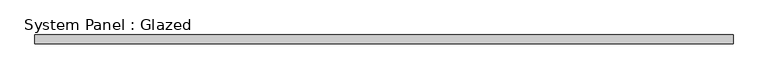
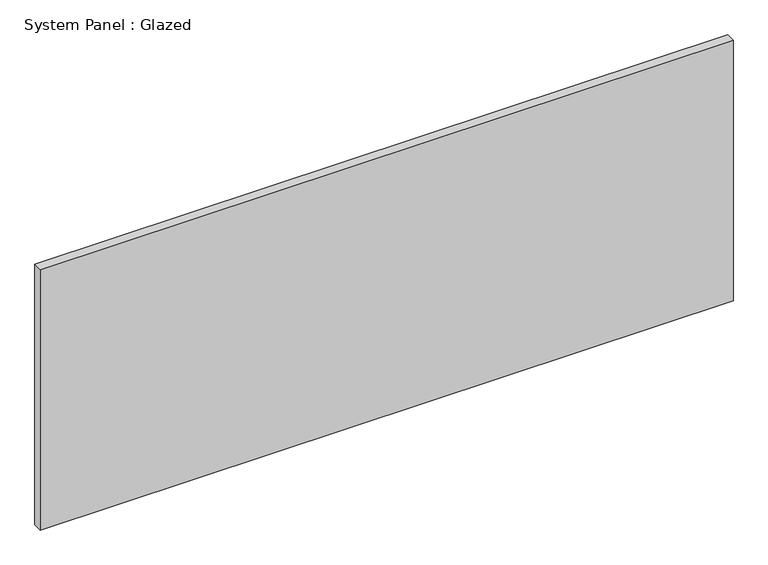
"""IFC4 building model written with IfcOpenShell, lengths in millimetres: plate geometry, System Panel : Glazed."""

import ifcopenshell
import ifcopenshell.guid

model = None  # the IFC model being written
_history = None  # IfcOwnerHistory: only IFC2X3 demands one
_inside = {}  # id of a spatial element -> (the spatial element, [elements in it])
_under = {}  # id of a project, library or spatial element -> (it, [spatial elements below it])
_declared = {}  # id of a project -> (the project, [libraries it declares])
_typed = {}  # id of a type object -> (the type object, [elements of that type])
_made_of = {}  # id of a material, layer set ... -> (it, [elements and type objects made of it])


def new_model(schema):
    """Start an empty IFC model of exactly this schema.

    Asked for "IFC4X3", IfcOpenShell would pick the latest addendum, in which some entities
    have other attributes; the version numbers below select the first issue.
    IFC2X3 requires an IfcOwnerHistory on every rooted entity: one is made here for all.
    """
    global model, _history
    if schema == "IFC4X3":
        model = ifcopenshell.file(schema_version=(4, 3, 0, 0))
    else:
        model = ifcopenshell.file(schema=schema)
    _inside.clear()
    _under.clear()
    _declared.clear()
    _typed.clear()
    _made_of.clear()
    _history = None
    if model.schema == "IFC2X3":
        org = make("IfcOrganization", Name="unknown")
        user = make(
            "IfcPersonAndOrganization",
            ThePerson=make("IfcPerson", FamilyName="unknown"),
            TheOrganization=org,
        )
        app = make(
            "IfcApplication",
            ApplicationDeveloper=org,
            Version="unknown",
            ApplicationFullName="unknown",
            ApplicationIdentifier="unknown",
        )
        _history = make(
            "IfcOwnerHistory",
            OwningUser=user,
            OwningApplication=app,
            ChangeAction="ADDED",
            CreationDate=0,
        )
    return model


def make(cls, **values):
    """One entity of the class cls with the attributes given. An attribute that is None is left unset."""
    return model.create_entity(
        cls, **{name: value for name, value in values.items() if value is not None}
    )


def rooted(cls, **values):
    """An entity with a GlobalId (a new one), such as an element, a storey or a relation."""
    return make(cls, GlobalId=ifcopenshell.guid.new(), OwnerHistory=_history, **values)


def si_unit(unit_type, name, prefix=None):
    """IfcSIUnit, for example si_unit("LENGTHUNIT", "METRE", prefix="MILLI")."""
    return make("IfcSIUnit", UnitType=unit_type, Prefix=prefix, Name=name)


def assignment(units):
    """IfcUnitAssignment: the units of a project."""
    return None if units is None else make("IfcUnitAssignment", Units=units)


def point(xyz):
    """IfcCartesianPoint."""
    return None if xyz is None else make("IfcCartesianPoint", Coordinates=xyz)


def direction(xyz):
    """IfcDirection."""
    return None if xyz is None else make("IfcDirection", DirectionRatios=xyz)


def frame(location, z_axis=None, x_axis=None):
    """IfcAxis2Placement3D, a coordinate frame: its origin and axes. An axis left out is left unset."""
    return make(
        "IfcAxis2Placement3D",
        Location=point(location),
        Axis=direction(z_axis),
        RefDirection=direction(x_axis),
    )


def origin():
    """The frame at (0, 0, 0) with its axes left unset."""
    return frame((0.0, 0.0, 0.0))


def origin_with_axes():
    """The frame at (0, 0, 0) with the z axis (0, 0, 1) and the x axis (1, 0, 0) written out."""
    return frame((0.0, 0.0, 0.0), z_axis=(0.0, 0.0, 1.0), x_axis=(1.0, 0.0, 0.0))


def place(relative_to, where):
    """IfcLocalPlacement: puts the frame where relative to a parent placement (None: the world)."""
    return make(
        "IfcLocalPlacement", PlacementRelTo=relative_to, RelativePlacement=where
    )


def context(
    kind, dimensions, precision=None, world=None, true_north=None, identifier=None
):
    """IfcGeometricRepresentationContext, for example the 3D "Model" context."""
    return make(
        "IfcGeometricRepresentationContext",
        ContextIdentifier=identifier,
        ContextType=kind,
        CoordinateSpaceDimension=dimensions,
        Precision=precision,
        WorldCoordinateSystem=world,
        TrueNorth=true_north,
    )


def project(units=None, contexts=None):
    """IfcProject with its units and contexts."""
    return rooted(
        "IfcProject",
        Name="project",
        RepresentationContexts=contexts,
        UnitsInContext=assignment(units),
    )


def spatial(cls, under=None, at=None, **own):
    """A site, building, storey or space (cls), placed at a placement, below another one or the project."""
    s = rooted(cls, ObjectPlacement=at, **own)
    if under is not None:
        _under.setdefault(under.id(), (under, []))[1].append(s)
    return s


def polyline(points):
    """IfcPolyline through the points."""
    return make("IfcPolyline", Points=[point(p) for p in points])


def outline(outer, holes=None, kind="AREA"):
    """IfcArbitraryClosedProfileDef: a profile drawn as a closed curve; with holes, ...WithVoids."""
    if holes is None:
        return make("IfcArbitraryClosedProfileDef", ProfileType=kind, OuterCurve=outer)
    return make(
        "IfcArbitraryProfileDefWithVoids",
        ProfileType=kind,
        OuterCurve=outer,
        InnerCurves=holes,
    )


def extrude(swept, where, along, depth):
    """IfcExtrudedAreaSolid: the profile swept, set in the frame where, extruded along a direction by depth."""
    return make(
        "IfcExtrudedAreaSolid",
        SweptArea=swept,
        Position=where,
        ExtrudedDirection=direction(along),
        Depth=depth,
    )


def shape(context_of_items, identifier, shape_type, items):
    """IfcShapeRepresentation: the items that make up one representation, for example the "Body"."""
    return make(
        "IfcShapeRepresentation",
        ContextOfItems=context_of_items,
        RepresentationIdentifier=identifier,
        RepresentationType=shape_type,
        Items=items,
    )


def source(mapping_origin, context_of_items, identifier, shape_type, items):
    """IfcRepresentationMap: a shape defined once, which mapped items show again and again."""
    return make(
        "IfcRepresentationMap",
        MappingOrigin=mapping_origin,
        MappedRepresentation=shape(context_of_items, identifier, shape_type, items),
    )


def transform(
    local_origin,
    x_axis=None,
    y_axis=None,
    z_axis=None,
    scale=None,
    scale2=None,
    scale3=None,
    uniform=True,
):
    """IfcCartesianTransformationOperator3D, or its non-uniform kind. x_axis, y_axis, z_axis: its Axis1, 2, 3."""
    if uniform:
        return make(
            "IfcCartesianTransformationOperator3D",
            Axis1=direction(x_axis),
            Axis2=direction(y_axis),
            LocalOrigin=point(local_origin),
            Scale=scale,
            Axis3=direction(z_axis),
        )
    return make(
        "IfcCartesianTransformationOperator3DnonUniform",
        Axis1=direction(x_axis),
        Axis2=direction(y_axis),
        LocalOrigin=point(local_origin),
        Scale=scale,
        Axis3=direction(z_axis),
        Scale2=scale2,
        Scale3=scale3,
    )


def mapped(mapping_source, mapping_target):
    """IfcMappedItem: shows the shape of a source again, moved by a transform."""
    return make(
        "IfcMappedItem", MappingSource=mapping_source, MappingTarget=mapping_target
    )


def made_of(thing, what):
    """Note that an element or type object is made of a material, layer set ...; save() writes the relation."""
    if what is not None:
        _made_of.setdefault(what.id(), (what, []))[1].append(thing)
    return thing


def element(
    cls,
    number,
    at=None,
    inside=None,
    cuts=None,
    type_object=None,
    material=None,
    context=None,
    identifier="Body",
    shape_type=None,
    held_by="IfcProductDefinitionShape",
    body=None,
    shapes=None,
    **own,
):
    """One element of the class cls, such as IfcWall. Its Tag is "e" and its number.

    at: its placement. inside: the storey or other place that contains it. cuts: it is an
    opening in that element (IfcRelVoidsElement). A single representation is given by context,
    identifier, shape_type and body (its items); several are given by shapes. held_by: the class
    of the entity that holds the representations. save() writes the other relations.
    """
    e = rooted(cls, Tag="e%d" % number, ObjectPlacement=at, **own)
    if body is not None:
        shapes = [shape(context, identifier, shape_type, body)]
    if shapes is not None:
        e.Representation = make(held_by, Representations=shapes)
    if inside is not None:
        _inside.setdefault(inside.id(), (inside, []))[1].append(e)
    if cuts is not None:
        rooted(
            "IfcRelVoidsElement", RelatingBuildingElement=cuts, RelatedOpeningElement=e
        )
    if type_object is not None:
        _typed.setdefault(type_object.id(), (type_object, []))[1].append(e)
    return made_of(e, material)


def aggregate(whole, parts):
    """IfcRelAggregates: a whole, such as a stair, and the parts it consists of."""
    return rooted("IfcRelAggregates", RelatingObject=whole, RelatedObjects=parts)


def save(model, path):
    """Write the relations noted so far, then the file.

    IfcRelAggregates (storeys below a building ...), IfcRelContainedInSpatialStructure (elements
    in a storey), IfcRelDefinesByType, IfcRelAssociatesMaterial and IfcRelDeclares: one each for
    every whole, place, type object, material and project.
    """
    for whole, parts in _under.values():
        aggregate(whole, parts)
    for where, things in _inside.values():
        rooted(
            "IfcRelContainedInSpatialStructure",
            RelatedElements=things,
            RelatingStructure=where,
        )
    for kind, things in _typed.values():
        rooted("IfcRelDefinesByType", RelatedObjects=things, RelatingType=kind)
    for what, things in _made_of.values():
        rooted("IfcRelAssociatesMaterial", RelatedObjects=things, RelatingMaterial=what)
    for by, libraries in _declared.values():
        rooted("IfcRelDeclares", RelatingContext=by, RelatedDefinitions=libraries)
    model.write(path)


def system_panel_glazed_d82c9dbb(model_context):
    return source(origin(), model_context, "Body", "SweptSolid", [
        extrude(outline(polyline([(975.0000002, 24.5), (-975.0000002, 24.5), (-975.0000002, 49.5), (975.0000002, 49.5), (975.0000002, 24.5)])), origin_with_axes(), (0.0, 0.0, 1.0), 775.0),
    ])


if __name__ == "__main__":
    model = new_model("IFC4")
    model_context = context("Model", 3, world=origin())
    ifc_project = project(units=[si_unit("LENGTHUNIT", "METRE", prefix="MILLI")], contexts=[model_context])
    site = spatial("IfcSite", under=ifc_project)
    building = spatial("IfcBuilding", under=site)
    placement = place(None, origin())
    system_panel_glazed_shape = system_panel_glazed_d82c9dbb(model_context)
    element("IfcPlate", 1, ObjectType="System Panel : Glazed", at=placement, inside=building, context=model_context, shape_type="MappedRepresentation", body=[
        mapped(system_panel_glazed_shape, transform((0.0, 0.0, 0.0), x_axis=(1.0, 0.0, 0.0), y_axis=(0.0, 1.0, 0.0), z_axis=(0.0, 0.0, 1.0))),
    ])
    save(model, "model.ifc")

# Revit data of these elements
# Element 1 (IfcPlate, "System Panel : Glazed")
#   Materials on its faces: "Glass"
# Materials
#   "Glass": class "Glass", colour RGB 0 128 192, transparency 0.9
